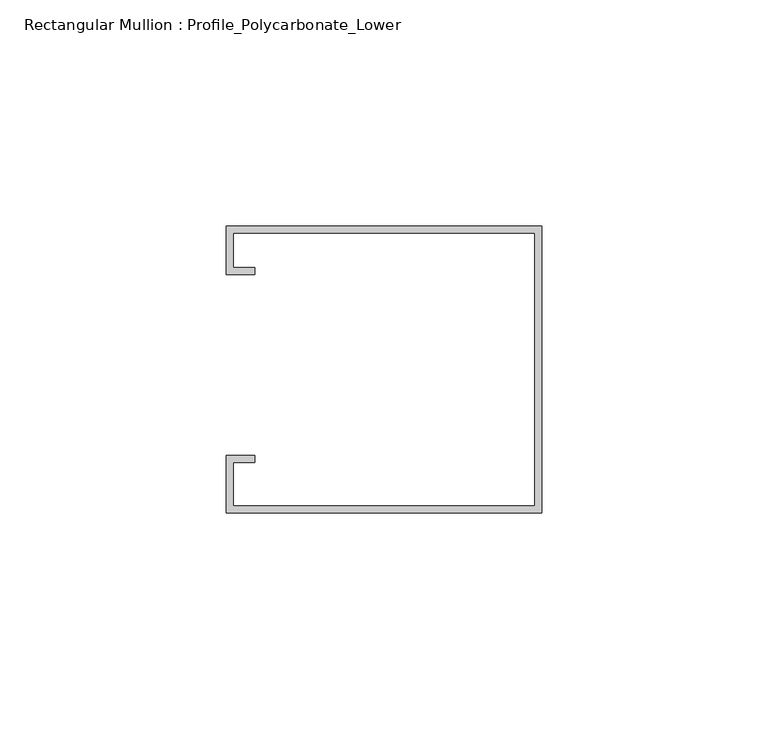
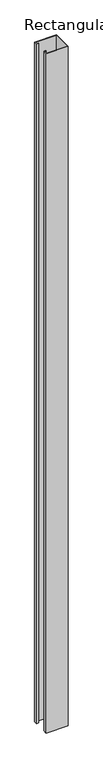
"""IFC4 building model written with IfcOpenShell, lengths in millimetres: member geometry, Rectangular Mullion : Profile_Polycarbonate_Lower."""

from ifc_helpers import new_model, si_unit, frame, origin, place, context, project, spatial, polyline, outline, extrude, source, transform, mapped, element, save


def rectangular_mullion_profile_polycarbonate_lower_fe93c9ce(model_context):
    return source(origin(), model_context, "Body", "SweptSolid", [
        extrude(outline(polyline([(0.0, -32.7), (-69.85, -32.7), (-69.85, -20.0), (-63.5, -20.0), (-63.5, -21.5875), (-68.2625, -21.5875), (-68.2625, -31.1125), (-1.5875, -31.1125), (-1.5875, 29.2125), (-68.2625, 29.2125), (-68.2625, 21.5875), (-63.5, 21.5875), (-63.5, 20.0), (-69.85, 20.0), (-69.85, 30.8), (0.0, 30.8), (0.0, -32.7)])), frame((0.0, 0.0, -2283.455133), z_axis=(0.0, 0.0, 1.0), x_axis=(1.0, 0.0, 0.0)), (0.0, 0.0, 1.0), 2283.455133),
    ])


if __name__ == "__main__":
    model = new_model("IFC4")
    model_context = context("Model", 3, world=origin())
    ifc_project = project(units=[si_unit("LENGTHUNIT", "METRE", prefix="MILLI")], contexts=[model_context])
    site = spatial("IfcSite", under=ifc_project)
    building = spatial("IfcBuilding", under=site)
    placement = place(None, origin())
    rectangular_mullion_profile_polycarbonate_lower_shape = rectangular_mullion_profile_polycarbonate_lower_fe93c9ce(model_context)
    element("IfcMember", 1, ObjectType="Rectangular Mullion : Profile_Polycarbonate_Lower", at=placement, inside=building, context=model_context, shape_type="MappedRepresentation", body=[
        mapped(rectangular_mullion_profile_polycarbonate_lower_shape, transform((0.0, 0.0, 0.0), x_axis=(1.0, 0.0, 0.0), y_axis=(0.0, 1.0, 0.0), z_axis=(0.0, 0.0, 1.0))),
    ])
    save(model, "model.ifc")

# Revit data of these elements
# Type "Rectangular Mullion : Profile_Polycarbonate_Lower"
#   built-in parameter 1007322 = 0.208333 (stored number, unit not read)
#   built-in parameter 1007321 = 0 (stored number, unit not read)
#   built-in parameter 1007320 = 0.00520833 (stored number, unit not read)
# Element 1 (IfcMember, "Rectangular Mullion : Profile_Polycarbonate_Lower")
#   Materials on its faces: "ALUMINUM PROFILE AT POLYCARBONATE PANEL"
# Materials
#   "ALUMINUM PROFILE AT POLYCARBONATE PANEL": class "Metal", colour RGB 244 244 244, transparency 0, Description = "Aluminum 6061", Cost = 0
